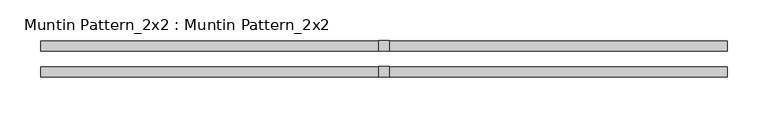
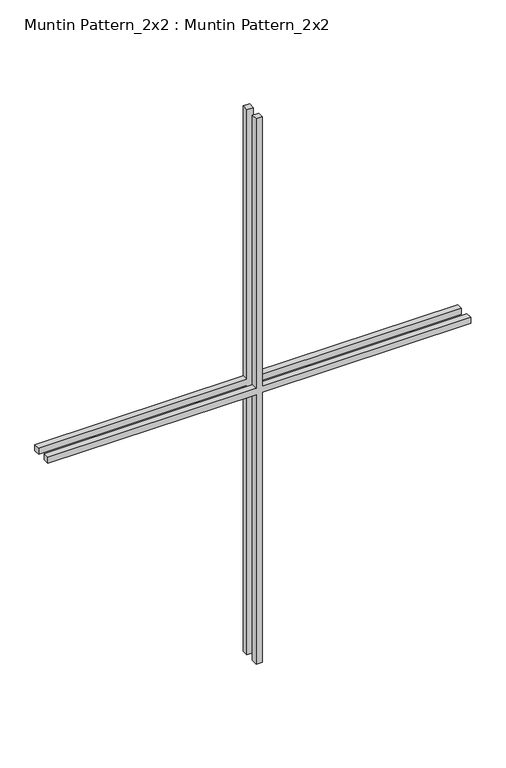
"""IFC4 building model written with IfcOpenShell, lengths in millimetres: proxy geometry, Muntin Pattern_2x2 : Muntin Pattern_2x2."""

from ifc_helpers import new_model, si_unit, frame, origin, place, context, project, spatial, polyline, outline, extrude, source, transform, mapped, element, save


def muntin_pattern_2x2_muntin_pattern_2x2_a23de983(model_context):
    return source(origin(), model_context, "Body", "SweptSolid", [
        extrude(outline(polyline([(577.85, -6.35), (577.85, -419.1), (565.15, -419.1), (565.15, -6.35), (0.0, -6.35), (0.0, 6.35), (565.15, 6.35), (565.15, 419.1), (577.85, 419.1), (577.85, 6.35), (1143.0, 6.35), (1143.0, -6.35), (577.85, -6.35)])), frame((0.0, 9.525, 0.0), z_axis=(0.0, 1.0, 0.0), x_axis=(0.0, 0.0, 1.0)), (0.0, 0.0, 1.0), 12.7),
        extrude(outline(polyline([(577.85, -6.35), (577.85, -419.1), (565.15, -419.1), (565.15, -6.35), (0.0, -6.35), (0.0, 6.35), (565.15, 6.35), (565.15, 419.1), (577.85, 419.1), (577.85, 6.35), (1143.0, 6.35), (1143.0, -6.35), (577.85, -6.35)])), frame((0.0, -22.225, 0.0), z_axis=(0.0, 1.0, 0.0), x_axis=(0.0, 0.0, 1.0)), (0.0, 0.0, 1.0), 12.7),
    ])


if __name__ == "__main__":
    model = new_model("IFC4")
    model_context = context("Model", 3, world=origin())
    ifc_project = project(units=[si_unit("LENGTHUNIT", "METRE", prefix="MILLI")], contexts=[model_context])
    site = spatial("IfcSite", under=ifc_project)
    building = spatial("IfcBuilding", under=site)
    placement = place(None, origin())
    muntin_pattern_2x2_muntin_pattern_2x2_shape = muntin_pattern_2x2_muntin_pattern_2x2_a23de983(model_context)
    element("IfcBuildingElementProxy", 1, Name="Muntin Pattern_2x2 : Muntin Pattern_2x2", ObjectType="Muntin Pattern_2x2 : Muntin Pattern_2x2", at=placement, inside=building, context=model_context, shape_type="MappedRepresentation", body=[
        mapped(muntin_pattern_2x2_muntin_pattern_2x2_shape, transform((0.0, 0.0, 0.0), x_axis=(1.0, 0.0, 0.0), y_axis=(0.0, 1.0, 0.0), z_axis=(0.0, 0.0, 1.0))),
    ])
    save(model, "model.ifc")

# Revit data of these elements
# Type "Muntin Pattern_2x2 : Muntin Pattern_2x2"
#   Width [instance default] = 4' - 0"
#   Thickness = 0' - 0 1/2"
#   Height [instance default] = 4' - 0"
#   Distance = 0' - 0 3/4"
#   Interior Material [instance default] = none
#   Exterior Material [instance default] = none
#   Default Elevation = 0
# Element 1 (IfcBuildingElementProxy, "Muntin Pattern_2x2 : Muntin Pattern_2x2")
#   Width = 2' - 9"
#   Height = 3' - 9"
#   Interior Material = Wood - Stained
#   Exterior Material = Clad - White
#   Materials on its faces: "Clad - White", "Wood - Stained"
# Materials
#   "Clad - White": class "Wood", colour RGB 242 242 238, transparency 0, Cost = 0
#   "Wood - Stained": class "Wood", colour RGB 224 178 126, transparency 0, Cost = 0
